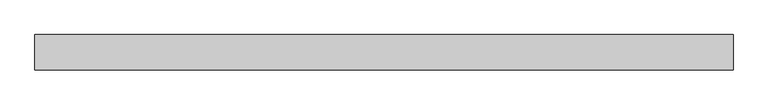
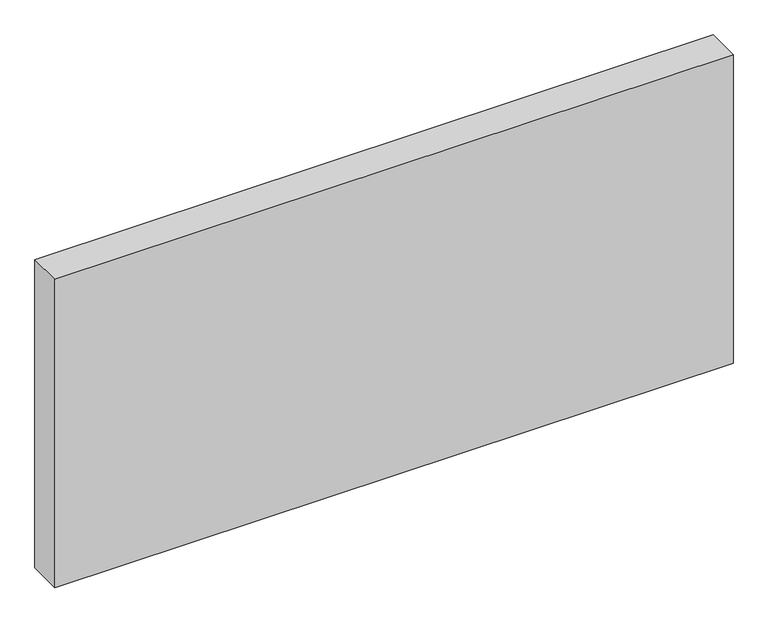
"""IFC4 building model written with IfcOpenShell, lengths in millimetres: proxy geometry, Generic Models 7:Generic Models 1:2:Generic Models 1:2 : Generic Models 7:Generic Models 1:337419:5 : Generic Models 7:Generic Models 1:2:Generic Models 1:2 : Generic Models 7:Generic Models 1:337419:306751."""

from ifc_helpers import new_model, si_unit, frame, origin, place, context, project, spatial, polyline, outline, extrude, source, transform, mapped, element, save


def generic_models_917ab4b2(model_context):
    return source(origin(), model_context, "Body", "SweptSolid", [
        extrude(outline(polyline([(596182.8367242, -567935.4195091), (596182.8367242, -568183.8632591), (591306.0367242, -568183.8632591), (591306.0367242, -567935.4195091), (596182.8367242, -567935.4195091)])), frame((0.0, 0.0, 2550.7278975), z_axis=(0.0, 0.0, 1.0), x_axis=(1.0, 0.0, 0.0)), (0.0, 0.0, 1.0), 2343.8784979),
    ])


if __name__ == "__main__":
    model = new_model("IFC4")
    model_context = context("Model", 3, world=origin())
    ifc_project = project(units=[si_unit("LENGTHUNIT", "METRE", prefix="MILLI")], contexts=[model_context])
    site = spatial("IfcSite", under=ifc_project)
    building = spatial("IfcBuilding", under=site)
    placement = place(None, origin())
    generic_models_shape = generic_models_917ab4b2(model_context)
    element("IfcBuildingElementProxy", 1, Name="Generic Models 7:Generic Models 1:2:Generic Models 1:2 : Generic Models 7:Generic Models 1:337419:5 : Generic Models 7:Generic Models 1:2:Generic Models 1:2 : Generic Models 7:Generic Models 1:337419:306751", ObjectType="Generic Models 7:Generic Models 1:2:Generic Models 1:2 : Generic Models 7:Generic Models 1:337419:5 : Generic Models 7:Generic Models 1:2:Generic Models 1:2 : Generic Models 7:Generic Models 1:337419:306751", at=placement, inside=building, context=model_context, shape_type="MappedRepresentation", body=[
        mapped(generic_models_shape, transform((0.0, 0.0, 0.0), x_axis=(1.0, 0.0, 0.0), y_axis=(0.0, 1.0, 0.0), z_axis=(0.0, 0.0, 1.0))),
    ])
    save(model, "model.ifc")

# Revit data of these elements
# Type "Generic Models 7:Generic Models 1:2:Generic Models 1:2 : Generic Models 7:Generic Models 1:337419:5 : Generic Models 7:Generic Models 1:2:Generic Models 1:2 : Generic Models 7:Generic Models 1:337419:306751"
#   NameOverride = "Generic Models 7:Generic Models 1:2:Generic Models 1:2 : Generic Models 7:Generic Models 1:337419:306751"
#   ObjectTypeOverride = "Generic Models 1:2 : Generic Models 7:Generic Models 1:337419"
#   Reference = "Generic Models 1"
#   Tag = "306751"
# Element 1 (IfcBuildingElementProxy, "Generic Models 7:Generic Models 1:2:Generic Models 1:2 : Generic Models 7:Generic Models 1:337419:5 : Generic Models 7:Generic Models 1:2:Generic Models 1:2 : Generic Models 7:Generic Models 1:337419:306751")
#   Materials on its faces: "FULL CAVITY CLASS A FIBERGLASS INSULATION WITH DURABLE VAPOR BARRIER (BLACK) LINER"
# Materials
#   "FULL CAVITY CLASS A FIBERGLASS INSULATION WITH DURABLE VAPOR BARRIER (BLACK) LINER": class "Unassigned", colour RGB 158 92 175, transparency 0, Cost = 0
